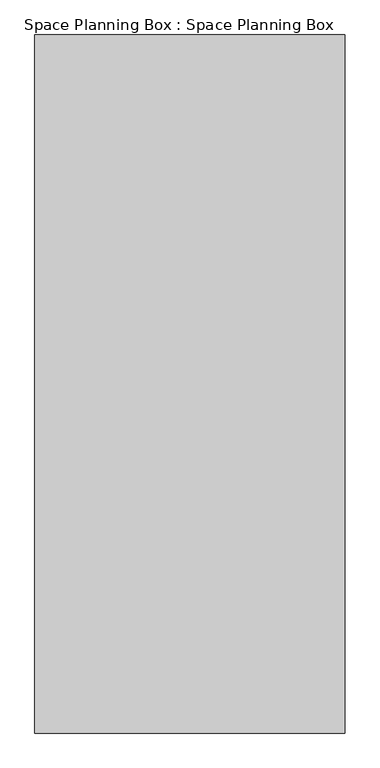
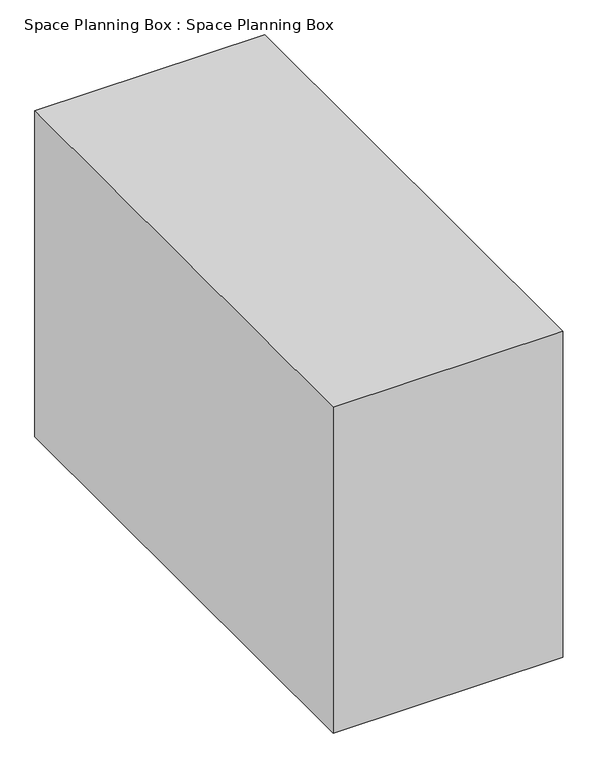
"""IFC4 building model written with IfcOpenShell, lengths in millimetres: proxy geometry, Space Planning Box : Space Planning Box."""

from ifc_helpers import new_model, si_unit, origin, origin_with_axes, place, context, project, spatial, polyline, outline, extrude, source, transform, mapped, element, save


def space_planning_box_space_planning_box_29bcd6f9(model_context):
    return source(origin(), model_context, "Body", "SweptSolid", [
        extrude(outline(polyline([(2000.0, 4500.0), (2000.0, -4500.0), (-2000.0, -4500.0), (-2000.0, 4500.0), (2000.0, 4500.0)])), origin_with_axes(), (0.0, 0.0, 1.0), 6000.0),
    ])


if __name__ == "__main__":
    model = new_model("IFC4")
    model_context = context("Model", 3, world=origin())
    ifc_project = project(units=[si_unit("LENGTHUNIT", "METRE", prefix="MILLI")], contexts=[model_context])
    site = spatial("IfcSite", under=ifc_project)
    building = spatial("IfcBuilding", under=site)
    placement = place(None, origin())
    space_planning_box_space_planning_box_shape = space_planning_box_space_planning_box_29bcd6f9(model_context)
    element("IfcBuildingElementProxy", 1, Name="Space Planning Box : Space Planning Box", ObjectType="Space Planning Box : Space Planning Box", at=placement, inside=building, context=model_context, shape_type="MappedRepresentation", body=[
        mapped(space_planning_box_space_planning_box_shape, transform((0.0, 0.0, 0.0), x_axis=(1.0, 0.0, 0.0), y_axis=(0.0, 1.0, 0.0), z_axis=(0.0, 0.0, 1.0))),
    ])
    save(model, "model.ifc")

# Revit data of these elements
# Type "Space Planning Box : Space Planning Box"
#   Type Comments = "..."
#   Room Name [instance default] = "?"
#   Assembly Code = "..."
#   Width [instance default] = 1524 mm
#   Program Area [instance default] = 0 m²
#   Length [instance default] = 1524 mm
#   Height [instance default] = 1524 mm
#   Area [instance default] = 2.32258 m²
#   Fill Color [instance default] = Cyan
#   Default Elevation = 0
# Element 1 (IfcBuildingElementProxy, "Space Planning Box : Space Planning Box")
#   Room Name = "Stairway"
#   Width = 4000 mm
#   Program Area = 36 m²
#   Length = 9000 mm
#   Height = 6000 mm
#   Area = 36 m²
#   Fill Color = Lavender
#   Materials on its faces: "Lavender"
# Materials
#   "Cyan": class "Generic", colour RGB 0 255 255, transparency 0.2, Cost = 0
#   "Lavender": class "Generic", colour RGB 186 85 211, transparency 0.2, Cost = 0
